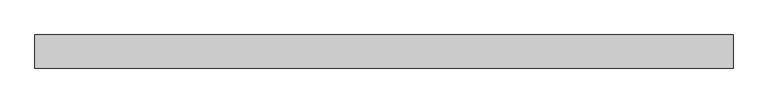
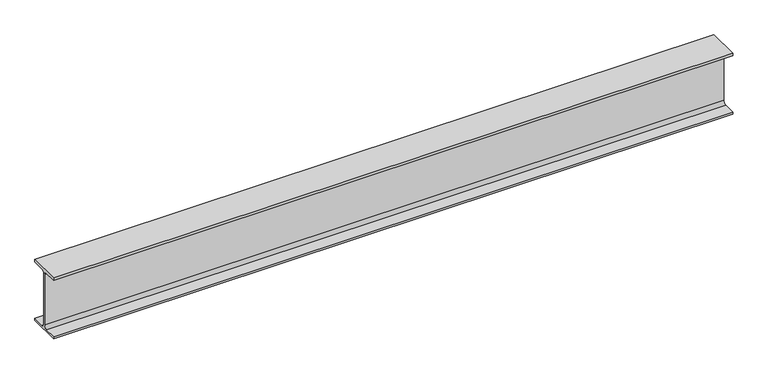
"""IFC4 building model written with IfcOpenShell, lengths in millimetres: beam geometry, 0912_Steel Framing_H-KSD3502 : H_SB_ASB_H-250x125x6x9."""

import ifcopenshell
import ifcopenshell.guid

model = None  # the IFC model being written
_history = None  # IfcOwnerHistory: only IFC2X3 demands one
_inside = {}  # id of a spatial element -> (the spatial element, [elements in it])
_under = {}  # id of a project, library or spatial element -> (it, [spatial elements below it])
_declared = {}  # id of a project -> (the project, [libraries it declares])
_typed = {}  # id of a type object -> (the type object, [elements of that type])
_made_of = {}  # id of a material, layer set ... -> (it, [elements and type objects made of it])


def new_model(schema):
    """Start an empty IFC model of exactly this schema.

    Asked for "IFC4X3", IfcOpenShell would pick the latest addendum, in which some entities
    have other attributes; the version numbers below select the first issue.
    IFC2X3 requires an IfcOwnerHistory on every rooted entity: one is made here for all.
    """
    global model, _history
    if schema == "IFC4X3":
        model = ifcopenshell.file(schema_version=(4, 3, 0, 0))
    else:
        model = ifcopenshell.file(schema=schema)
    _inside.clear()
    _under.clear()
    _declared.clear()
    _typed.clear()
    _made_of.clear()
    _history = None
    if model.schema == "IFC2X3":
        org = make("IfcOrganization", Name="unknown")
        user = make(
            "IfcPersonAndOrganization",
            ThePerson=make("IfcPerson", FamilyName="unknown"),
            TheOrganization=org,
        )
        app = make(
            "IfcApplication",
            ApplicationDeveloper=org,
            Version="unknown",
            ApplicationFullName="unknown",
            ApplicationIdentifier="unknown",
        )
        _history = make(
            "IfcOwnerHistory",
            OwningUser=user,
            OwningApplication=app,
            ChangeAction="ADDED",
            CreationDate=0,
        )
    return model


def make(cls, **values):
    """One entity of the class cls with the attributes given. An attribute that is None is left unset."""
    return model.create_entity(
        cls, **{name: value for name, value in values.items() if value is not None}
    )


def rooted(cls, **values):
    """An entity with a GlobalId (a new one), such as an element, a storey or a relation."""
    return make(cls, GlobalId=ifcopenshell.guid.new(), OwnerHistory=_history, **values)


def si_unit(unit_type, name, prefix=None):
    """IfcSIUnit, for example si_unit("LENGTHUNIT", "METRE", prefix="MILLI")."""
    return make("IfcSIUnit", UnitType=unit_type, Prefix=prefix, Name=name)


def assignment(units):
    """IfcUnitAssignment: the units of a project."""
    return None if units is None else make("IfcUnitAssignment", Units=units)


def point(xyz):
    """IfcCartesianPoint."""
    return None if xyz is None else make("IfcCartesianPoint", Coordinates=xyz)


def direction(xyz):
    """IfcDirection."""
    return None if xyz is None else make("IfcDirection", DirectionRatios=xyz)


def frame(location, z_axis=None, x_axis=None):
    """IfcAxis2Placement3D, a coordinate frame: its origin and axes. An axis left out is left unset."""
    return make(
        "IfcAxis2Placement3D",
        Location=point(location),
        Axis=direction(z_axis),
        RefDirection=direction(x_axis),
    )


def frame_2d(location, x_axis=None):
    """IfcAxis2Placement2D, a coordinate frame in the plane: its origin and x axis."""
    return make(
        "IfcAxis2Placement2D", Location=point(location), RefDirection=direction(x_axis)
    )


def origin():
    """The frame at (0, 0, 0) with its axes left unset."""
    return frame((0.0, 0.0, 0.0))


def place(relative_to, where):
    """IfcLocalPlacement: puts the frame where relative to a parent placement (None: the world)."""
    return make(
        "IfcLocalPlacement", PlacementRelTo=relative_to, RelativePlacement=where
    )


def context(
    kind, dimensions, precision=None, world=None, true_north=None, identifier=None
):
    """IfcGeometricRepresentationContext, for example the 3D "Model" context."""
    return make(
        "IfcGeometricRepresentationContext",
        ContextIdentifier=identifier,
        ContextType=kind,
        CoordinateSpaceDimension=dimensions,
        Precision=precision,
        WorldCoordinateSystem=world,
        TrueNorth=true_north,
    )


def project(units=None, contexts=None):
    """IfcProject with its units and contexts."""
    return rooted(
        "IfcProject",
        Name="project",
        RepresentationContexts=contexts,
        UnitsInContext=assignment(units),
    )


def spatial(cls, under=None, at=None, **own):
    """A site, building, storey or space (cls), placed at a placement, below another one or the project."""
    s = rooted(cls, ObjectPlacement=at, **own)
    if under is not None:
        _under.setdefault(under.id(), (under, []))[1].append(s)
    return s


def polyline(points):
    """IfcPolyline through the points."""
    return make("IfcPolyline", Points=[point(p) for p in points])


def circle_curve(where, radius):
    """IfcCircle in the frame where."""
    return make("IfcCircle", Position=where, Radius=radius)


def trimmed(basis, trim1, trim2, sense, master):
    """IfcTrimmedCurve: the piece of a basis curve between two trims."""
    return make(
        "IfcTrimmedCurve",
        BasisCurve=basis,
        Trim1=trim1,
        Trim2=trim2,
        SenseAgreement=sense,
        MasterRepresentation=master,
    )


def segment(curve, same_sense, transition):
    """IfcCompositeCurveSegment."""
    return make(
        "IfcCompositeCurveSegment",
        Transition=transition,
        SameSense=same_sense,
        ParentCurve=curve,
    )


def composite_curve(segments, self_intersect=None):
    """IfcCompositeCurve: segments joined end to end."""
    return make("IfcCompositeCurve", Segments=segments, SelfIntersect=self_intersect)


def outline(outer, holes=None, kind="AREA"):
    """IfcArbitraryClosedProfileDef: a profile drawn as a closed curve; with holes, ...WithVoids."""
    if holes is None:
        return make("IfcArbitraryClosedProfileDef", ProfileType=kind, OuterCurve=outer)
    return make(
        "IfcArbitraryProfileDefWithVoids",
        ProfileType=kind,
        OuterCurve=outer,
        InnerCurves=holes,
    )


def extrude(swept, where, along, depth):
    """IfcExtrudedAreaSolid: the profile swept, set in the frame where, extruded along a direction by depth."""
    return make(
        "IfcExtrudedAreaSolid",
        SweptArea=swept,
        Position=where,
        ExtrudedDirection=direction(along),
        Depth=depth,
    )


def shape(context_of_items, identifier, shape_type, items):
    """IfcShapeRepresentation: the items that make up one representation, for example the "Body"."""
    return make(
        "IfcShapeRepresentation",
        ContextOfItems=context_of_items,
        RepresentationIdentifier=identifier,
        RepresentationType=shape_type,
        Items=items,
    )


def source(mapping_origin, context_of_items, identifier, shape_type, items):
    """IfcRepresentationMap: a shape defined once, which mapped items show again and again."""
    return make(
        "IfcRepresentationMap",
        MappingOrigin=mapping_origin,
        MappedRepresentation=shape(context_of_items, identifier, shape_type, items),
    )


def transform(
    local_origin,
    x_axis=None,
    y_axis=None,
    z_axis=None,
    scale=None,
    scale2=None,
    scale3=None,
    uniform=True,
):
    """IfcCartesianTransformationOperator3D, or its non-uniform kind. x_axis, y_axis, z_axis: its Axis1, 2, 3."""
    if uniform:
        return make(
            "IfcCartesianTransformationOperator3D",
            Axis1=direction(x_axis),
            Axis2=direction(y_axis),
            LocalOrigin=point(local_origin),
            Scale=scale,
            Axis3=direction(z_axis),
        )
    return make(
        "IfcCartesianTransformationOperator3DnonUniform",
        Axis1=direction(x_axis),
        Axis2=direction(y_axis),
        LocalOrigin=point(local_origin),
        Scale=scale,
        Axis3=direction(z_axis),
        Scale2=scale2,
        Scale3=scale3,
    )


def mapped(mapping_source, mapping_target):
    """IfcMappedItem: shows the shape of a source again, moved by a transform."""
    return make(
        "IfcMappedItem", MappingSource=mapping_source, MappingTarget=mapping_target
    )


def made_of(thing, what):
    """Note that an element or type object is made of a material, layer set ...; save() writes the relation."""
    if what is not None:
        _made_of.setdefault(what.id(), (what, []))[1].append(thing)
    return thing


def element(
    cls,
    number,
    at=None,
    inside=None,
    cuts=None,
    type_object=None,
    material=None,
    context=None,
    identifier="Body",
    shape_type=None,
    held_by="IfcProductDefinitionShape",
    body=None,
    shapes=None,
    **own,
):
    """One element of the class cls, such as IfcWall. Its Tag is "e" and its number.

    at: its placement. inside: the storey or other place that contains it. cuts: it is an
    opening in that element (IfcRelVoidsElement). A single representation is given by context,
    identifier, shape_type and body (its items); several are given by shapes. held_by: the class
    of the entity that holds the representations. save() writes the other relations.
    """
    e = rooted(cls, Tag="e%d" % number, ObjectPlacement=at, **own)
    if body is not None:
        shapes = [shape(context, identifier, shape_type, body)]
    if shapes is not None:
        e.Representation = make(held_by, Representations=shapes)
    if inside is not None:
        _inside.setdefault(inside.id(), (inside, []))[1].append(e)
    if cuts is not None:
        rooted(
            "IfcRelVoidsElement", RelatingBuildingElement=cuts, RelatedOpeningElement=e
        )
    if type_object is not None:
        _typed.setdefault(type_object.id(), (type_object, []))[1].append(e)
    return made_of(e, material)


def aggregate(whole, parts):
    """IfcRelAggregates: a whole, such as a stair, and the parts it consists of."""
    return rooted("IfcRelAggregates", RelatingObject=whole, RelatedObjects=parts)


def save(model, path):
    """Write the relations noted so far, then the file.

    IfcRelAggregates (storeys below a building ...), IfcRelContainedInSpatialStructure (elements
    in a storey), IfcRelDefinesByType, IfcRelAssociatesMaterial and IfcRelDeclares: one each for
    every whole, place, type object, material and project.
    """
    for whole, parts in _under.values():
        aggregate(whole, parts)
    for where, things in _inside.values():
        rooted(
            "IfcRelContainedInSpatialStructure",
            RelatedElements=things,
            RelatingStructure=where,
        )
    for kind, things in _typed.values():
        rooted("IfcRelDefinesByType", RelatedObjects=things, RelatingType=kind)
    for what, things in _made_of.values():
        rooted("IfcRelAssociatesMaterial", RelatedObjects=things, RelatingMaterial=what)
    for by, libraries in _declared.values():
        rooted("IfcRelDeclares", RelatingContext=by, RelatedDefinitions=libraries)
    model.write(path)


def beam_ec440c2a(model_context):
    return source(origin(), model_context, "Body", "SweptSolid", [
        extrude(outline(composite_curve([segment(polyline([(62.5, -116.0), (62.5, -125.0), (-62.5, -125.0), (-62.5, -116.0), (-15.0, -116.0)]), True, "CONTINUOUS"), segment(trimmed(circle_curve(frame_2d((-15.0, -104.0)), 12.0), [point((-15.0, -116.0))], [point((-3.0, -104.0))], True, "CARTESIAN"), True, "CONTINUOUS"), segment(polyline([(-3.0, -104.0), (-3.0, 104.0)]), True, "CONTINUOUS"), segment(trimmed(circle_curve(frame_2d((-15.0, 104.0)), 12.0), [point((-3.0, 104.0))], [point((-15.0, 116.0))], True, "CARTESIAN"), True, "CONTINUOUS"), segment(polyline([(-15.0, 116.0), (-62.5, 116.0), (-62.5, 125.0), (62.5, 125.0), (62.5, 116.0), (15.0, 116.0)]), True, "CONTINUOUS"), segment(trimmed(circle_curve(frame_2d((15.0, 104.0)), 12.0), [point((15.0, 116.0))], [point((3.0, 104.0))], True, "CARTESIAN"), True, "CONTINUOUS"), segment(polyline([(3.0, 104.0), (3.0, -104.0)]), True, "CONTINUOUS"), segment(trimmed(circle_curve(frame_2d((15.0, -104.0)), 12.0), [point((3.0, -104.0))], [point((15.0, -116.0))], True, "CARTESIAN"), True, "CONTINUOUS"), segment(polyline([(15.0, -116.0), (62.5, -116.0)]), True, "CONTINUOUS")], self_intersect=False)), frame((-1387.3, 0.0, 0.0), z_axis=(1.0, 0.0, 0.0), x_axis=(0.0, 1.0, 0.0)), (0.0, 0.0, 1.0), 2636.6),
    ])


if __name__ == "__main__":
    model = new_model("IFC4")
    model_context = context("Model", 3, world=origin())
    ifc_project = project(units=[si_unit("LENGTHUNIT", "METRE", prefix="MILLI")], contexts=[model_context])
    site = spatial("IfcSite", under=ifc_project)
    building = spatial("IfcBuilding", under=site)
    placement = place(None, origin())
    beam_shape = beam_ec440c2a(model_context)
    element("IfcBeam", 1, ObjectType="0912_Steel Framing_H-KSD3502 : H_SB_ASB_H-250x125x6x9", at=placement, inside=building, context=model_context, shape_type="MappedRepresentation", body=[
        mapped(beam_shape, transform((0.0, 0.0, 0.0), x_axis=(1.0, 0.0, 0.0), y_axis=(0.0, 1.0, 0.0), z_axis=(0.0, 0.0, 1.0))),
    ])
    save(model, "model.ifc")

# Revit data of these elements
# Type "0912_Steel Framing_H-KSD3502 : H_SB_ASB_H-250x125x6x9"
#   H_WM Code_1 = "S01AA003-00001 | Main Steel Structure Fabrication Work | Shelter/Building | Light Steel - Standard (30KG/M>Weight) | Material: (   )"
#   H_WM Code_2 = "S03AA029-00001 | Main Steel Structure Erection Work | Shelter/Building | Light Steel (30KG/M>Weight) | Material: (   )"
#   H_WM Code_3 = "S01AA010-00001 | Main Steel Structure Fabrication Work | Shelter/Building | Steel Painting/Coating | for Non-Fireproofed Steel Surface, Surface Preparation, Primer, Second & Final Coat | Material: (   )"
#   H_Q'ty Cal Type Tag = "SB-Q2"
#   Width = 12.5 cm
#   Web Thickness = 0.6 cm
#   Web Fillet = 1.2 cm
#   Warping Constant = 42539.8 cm⁶
#   W = 0
#   Torsional Moment of Inertia = 7.8102 cm⁴
#   Section Area = 37.66 cm²
#   Plastic Modulus weak axis = 73.1 cm³
#   Plastic Modulus strong axis = 366.0 cm³
#   Perimeter = 0.97 m²/m
#   Nominal Weight = 29.60 kgf/m
#   Moment of Inertia weak axis = 294.00 cm⁴
#   Moment of Inertia strong axis = 4050.00 cm⁴
#   Height = 25.0 cm
#   Flange Thickness = 0.9 cm
#   Elastic Modulus weak axis = 47.0 cm³
#   Elastic Modulus strong axis = 324.0 cm³
#   Centroid Vertical = 12.5 cm
#   Centroid Horizontal = 6.25 cm
#   Ix = 40500000
#   Length [instance default] = 1.5240 m
#   Zx = 366000
#   b = 0.1250 m
#   h = 0.2500 m
#   r = 0.0120 m
#   s = 0.0060 m
#   t = 0.0090 m
#   A = 0.003766 m²
#   Structural Material [instance default] = Steel, 45-345
#   Assembly Code = ""
# Element 1 (IfcBeam, "0912_Steel Framing_H-KSD3502 : H_SB_ASB_H-250x125x6x9")
#   Structural Material = none
# Materials
#   "Steel, 45-345": class "Metal", colour RGB 189 187 185, transparency 0, Description = "Steel 345 MPa", Cost = 0
